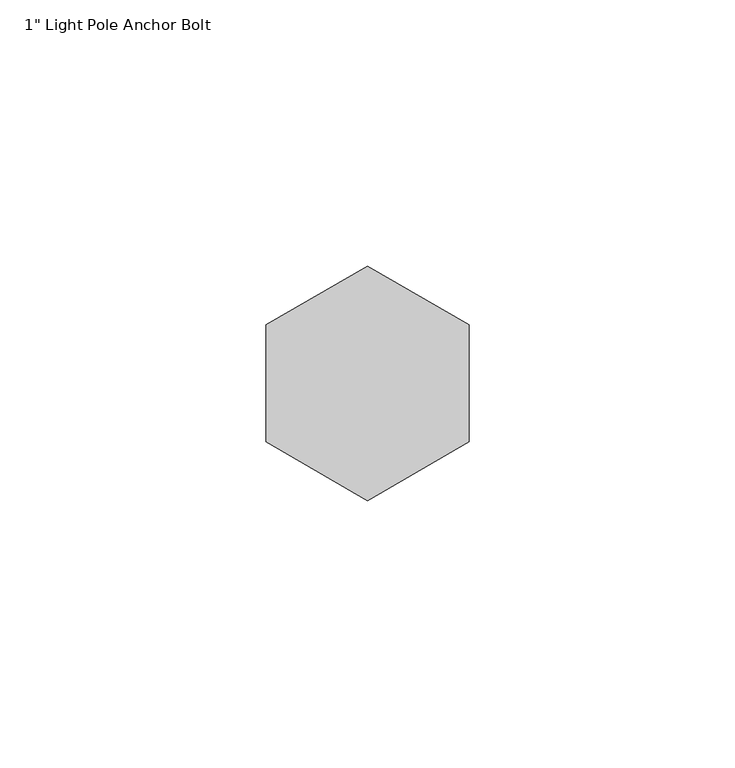
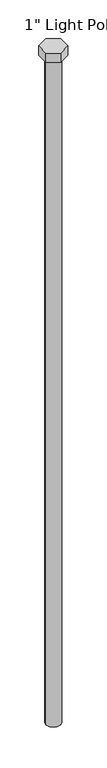
"""IFC4 building model written with IfcOpenShell, lengths in millimetres: proxy geometry."""

from ifc_helpers import new_model, si_unit, point, frame, origin, origin_with_axes, origin_2d, place, context, project, spatial, polyline, circle_curve, trimmed, segment, composite_curve, outline, extrude, source, transform, mapped, element, save


def proxy_e5fc580f(model_context):
    return source(origin(), model_context, "Body", "SweptSolid", [
        extrude(outline(polyline([(-19.05, 10.9985226), (0.0, 21.9970453), (19.05, 10.9985226), (19.05, -10.9985226), (0.0, -21.9970453), (-19.05, -10.9985226), (-19.05, 10.9985226)])), origin_with_axes(), (0.0, 0.0, 1.0), 17.065625),
        extrude(outline(composite_curve([segment(trimmed(circle_curve(origin_2d(), 12.7), [point((-12.7, 0.0))], [point((12.7, 0.0))], False, "CARTESIAN"), True, "CONTINUOUS"), segment(trimmed(circle_curve(origin_2d(), 12.7), [point((12.7, 0.0))], [point((-12.7, 0.0))], False, "CARTESIAN"), True, "CONTINUOUS")], self_intersect=False)), frame((0.0, 0.0, -1219.2), z_axis=(0.0, 0.0, 1.0), x_axis=(1.0, 0.0, 0.0)), (0.0, 0.0, 1.0), 1219.2),
    ])


if __name__ == "__main__":
    model = new_model("IFC4")
    model_context = context("Model", 3, world=origin())
    ifc_project = project(units=[si_unit("LENGTHUNIT", "METRE", prefix="MILLI")], contexts=[model_context])
    site = spatial("IfcSite", under=ifc_project)
    building = spatial("IfcBuilding", under=site)
    placement = place(None, origin())
    proxy_shape = proxy_e5fc580f(model_context)
    element("IfcBuildingElementProxy", 1, Name="050523 - W_P_C - Fastenings - Lag Bolt or Thru Bolt : 1\" Light Pole Anchor Bolt", ObjectType="050523 - W_P_C - Fastenings - Lag Bolt or Thru Bolt : 1\" Light Pole Anchor Bolt", at=placement, inside=building, context=model_context, shape_type="MappedRepresentation", body=[
        mapped(proxy_shape, transform((0.0, 0.0, 0.0), x_axis=(1.0, 0.0, 0.0), y_axis=(0.0, 1.0, 0.0), z_axis=(0.0, 0.0, 1.0))),
    ])
    save(model, "model.ifc")

# Revit data of these elements
# Type "050523 - W_P_C - Fastenings - Lag Bolt or Thru Bolt : 1\" Light Pole Anchor Bolt"
#   Thickness_of_Substrate [instance default] = 0' - 1"
#   Side = 0' - 0 111/128"
#   Radius = 0' - 0 1/2"
#   Length = 4' - 0"
#   Head Size = 0' - 1 1/2"
#   Head Radius = 0' - 0 3/4"
#   Head Height = 0' - 0 43/64"
#   Diameter = 0' - 1"
#   Default Elevation = 4' - 0"
#   Nut_Visibility [instance default] = yes
#   Bolt Material (Size) = (4) GALV. ANCHOR BOLTS - SUPPLIED W/ LIGHT POLE
# Element 1 (IfcBuildingElementProxy, "050523 - W_P_C - Fastenings - Lag Bolt or Thru Bolt : 1\" Light Pole Anchor Bolt")
#   Thickness_of_Substrate = 3' - 0"
#   Nut_Visibility = no
#   Materials on its faces: "(4) GALV. ANCHOR BOLTS - SUPPLIED W/ LIGHT POLE"
# Materials
#   "(4) GALV. ANCHOR BOLTS - SUPPLIED W/ LIGHT POLE": class "Generic", colour RGB 120 120 120, transparency 0, Cost = 0
